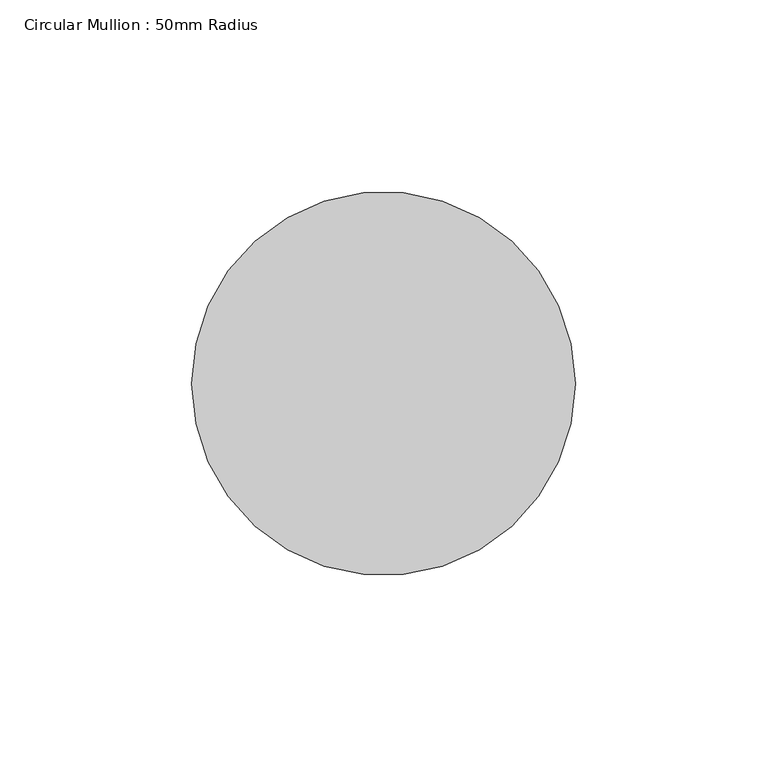
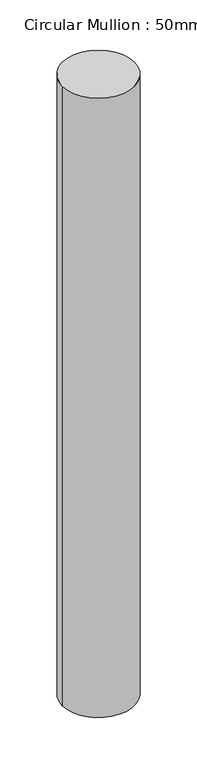
"""IFC4 building model written with IfcOpenShell, lengths in millimetres: member geometry, Circular Mullion : 50mm Radius."""

from ifc_helpers import new_model, si_unit, point, frame, origin, origin_2d, place, context, project, spatial, circle_curve, trimmed, segment, composite_curve, outline, extrude, source, transform, mapped, element, save


def circular_mullion_50mm_radius_df1f6790(model_context):
    return source(origin(), model_context, "Body", "SweptSolid", [
        extrude(outline(composite_curve([segment(trimmed(circle_curve(origin_2d(), 50.0), [point((50.0, 0.0))], [point((-50.0, 0.0))], False, "CARTESIAN"), True, "CONTINUOUS"), segment(trimmed(circle_curve(origin_2d(), 50.0), [point((-50.0, 0.0))], [point((50.0, 0.0))], False, "CARTESIAN"), True, "CONTINUOUS")], self_intersect=False)), frame((0.0, 0.0, -907.4315539), z_axis=(0.0, 0.0, 1.0), x_axis=(1.0, 0.0, 0.0)), (0.0, 0.0, 1.0), 907.4315539),
    ])


if __name__ == "__main__":
    model = new_model("IFC4")
    model_context = context("Model", 3, world=origin())
    ifc_project = project(units=[si_unit("LENGTHUNIT", "METRE", prefix="MILLI")], contexts=[model_context])
    site = spatial("IfcSite", under=ifc_project)
    building = spatial("IfcBuilding", under=site)
    placement = place(None, origin())
    circular_mullion_50mm_radius_shape = circular_mullion_50mm_radius_df1f6790(model_context)
    element("IfcMember", 1, ObjectType="Circular Mullion : 50mm Radius", at=placement, inside=building, context=model_context, shape_type="MappedRepresentation", body=[
        mapped(circular_mullion_50mm_radius_shape, transform((0.0, 0.0, 0.0), x_axis=(1.0, 0.0, 0.0), y_axis=(0.0, 1.0, 0.0), z_axis=(0.0, 0.0, 1.0))),
    ])
    save(model, "model.ifc")

# Revit data of these elements
# Type "Circular Mullion : 50mm Radius"
#   built-in parameter 1007350 = 0.164042 (stored number, unit not read)
# Element 1 (IfcMember, "Circular Mullion : 50mm Radius")
#   Materials on its faces: "Aluminium"
# Materials
#   "Aluminium": class "Metal", colour RGB 247 247 247, transparency 0, Description = "Aluminium 6061", Cost = 0
